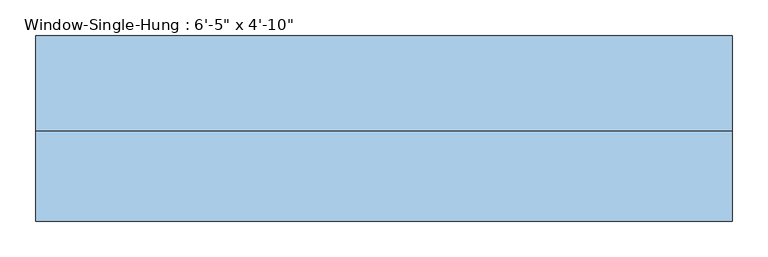
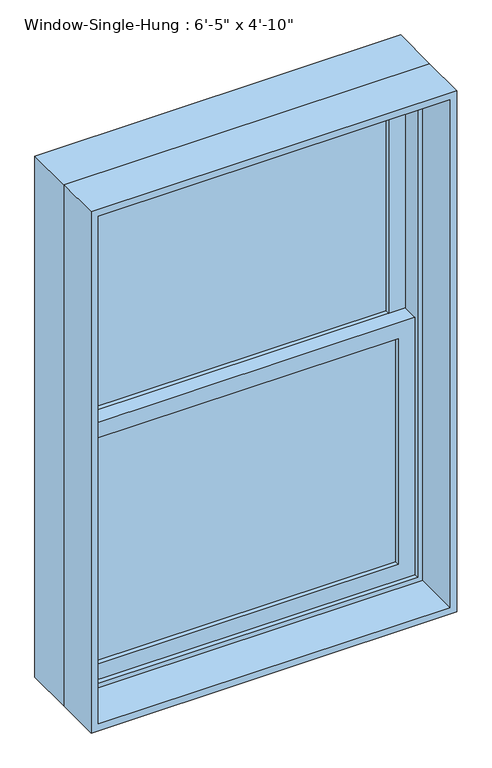
"""IFC4 building model written with IfcOpenShell, lengths in millimetres: window geometry."""

from ifc_helpers import new_model, si_unit, frame, origin, place, context, project, spatial, polyline, outline, extrude, source, transform, mapped, element, save


def window_979dede4(model_context):
    return source(origin(), model_context, "Body", "SweptSolid", [
        extrude(outline(polyline([(412.75, 50.8), (412.75, 44.45), (-412.75, 44.45), (-412.75, 50.8), (412.75, 50.8)])), frame((0.0, 0.0, 990.6), z_axis=(0.0, 0.0, 1.0), x_axis=(1.0, 0.0, 0.0)), (0.0, 0.0, 1.0), 638.175),
        extrude(outline(polyline([(-412.75, 38.1), (412.75, 38.1), (412.75, 31.75), (-412.75, 31.75), (-412.75, 38.1)])), frame((0.0, 0.0, 990.6), z_axis=(0.0, 0.0, 1.0), x_axis=(1.0, 0.0, 0.0)), (0.0, 0.0, 1.0), 638.175),
        extrude(outline(polyline([(412.75, 95.25), (412.75, 88.9), (-412.75, 88.9), (-412.75, 95.25), (412.75, 95.25)])), frame((0.0, 0.0, 1673.225), z_axis=(0.0, 0.0, 1.0), x_axis=(1.0, 0.0, 0.0)), (0.0, 0.0, 1.0), 638.175),
        extrude(outline(polyline([(-412.75, 82.55), (412.75, 82.55), (412.75, 76.2), (-412.75, 76.2), (-412.75, 82.55)])), frame((0.0, 0.0, 1673.225), z_axis=(0.0, 0.0, 1.0), x_axis=(1.0, 0.0, 0.0)), (0.0, 0.0, 1.0), 638.175),
        extrude(outline(polyline([(1673.225, -457.2), (946.15, -457.2), (946.15, 457.2), (1673.225, 457.2), (1673.225, -457.2)]), holes=[polyline([(1628.775, 412.75), (990.6, 412.75), (990.6, -412.75), (1628.775, -412.75), (1628.775, 412.75)])]), frame((0.0, 19.05, 0.0), z_axis=(0.0, 1.0, 0.0), x_axis=(0.0, 0.0, 1.0)), (0.0, 0.0, 1.0), 44.45),
        extrude(outline(polyline([(2355.85, -457.2), (1628.775, -457.2), (1628.775, 457.2), (2355.85, 457.2), (2355.85, -457.2)]), holes=[polyline([(2311.4, 412.75), (1673.225, 412.75), (1673.225, -412.75), (2311.4, -412.75), (2311.4, 412.75)])]), frame((0.0, 63.5, 0.0), z_axis=(0.0, 1.0, 0.0), x_axis=(0.0, 0.0, 1.0)), (0.0, 0.0, 1.0), 44.45),
        extrude(outline(polyline([(2387.6, -488.95), (914.4, -488.95), (914.4, 488.95), (2387.6, 488.95), (2387.6, -488.95)]), holes=[polyline([(2355.85, 457.2), (946.15, 457.2), (946.15, -457.2), (2355.85, -457.2), (2355.85, 457.2)])]), frame((0.0, 6.35, 0.0), z_axis=(0.0, 1.0, 0.0), x_axis=(0.0, 0.0, 1.0)), (0.0, 0.0, 1.0), 133.35),
        extrude(outline(polyline([(2387.6, 488.95), (2387.6, -488.95), (914.4, -488.95), (914.4, 488.95), (2387.6, 488.95)]), holes=[polyline([(2368.55, 469.9), (933.45, 469.9), (933.45, -469.9), (2368.55, -469.9), (2368.55, 469.9)])]), frame((0.0, -120.65, 0.0), z_axis=(0.0, 1.0, 0.0), x_axis=(0.0, 0.0, 1.0)), (0.0, 0.0, 1.0), 127.0),
    ])


if __name__ == "__main__":
    model = new_model("IFC4")
    model_context = context("Model", 3, world=origin())
    ifc_project = project(units=[si_unit("LENGTHUNIT", "METRE", prefix="MILLI")], contexts=[model_context])
    site = spatial("IfcSite", under=ifc_project)
    building = spatial("IfcBuilding", under=site)
    placement = place(None, origin())
    window_shape = window_979dede4(model_context)
    element("IfcWindow", 1, ObjectType="Window-Single-Hung : 6'-5\" x 4'-10\"", at=placement, inside=building, context=model_context, shape_type="MappedRepresentation", body=[
        mapped(window_shape, transform((0.0, 0.0, 0.0), x_axis=(1.0, 0.0, 0.0), y_axis=(0.0, 1.0, 0.0), z_axis=(0.0, 0.0, 1.0))),
    ])
    save(model, "model.ifc")

# Revit data of these elements
# Type "Window-Single-Hung : 6'-5\" x 4'-10\""
#   Type Mark = "19"
#   Fire Rating = "0.5h"
#   Construction Type Id = "DG-DR"
#   Assembly Code = "B2020100"
#   Analytic Construction = "Double glazing - domestic"
#   Wall Thickness [instance default] = 0' - 6"
#   Window Inset [instance default] = 0' - 0"
#   Visual Light Transmittance = 0.81
#   Thermal Resistance (R) = 0.319569 (m²·K)/W
#   Solar Heat Gain Coefficient = 0.76
#   Muntin Width = 2' - 8 1/2"
#   Muntin Height = 2' - 1 1/8"
#   Interior Wall Closure [instance default] = 0' - 1 1/2"
#   Rough Width = 3' - 3"
#   Rough Height = 4' - 10 1/2"
#   Frame Extension [instance default] = 0' - 1 1/4"
#   Exterior Wall Closure [instance default] = 0' - 0 1/2"
#   Extension Jamb [instance default] = 0' - 1 1/2"
#   Heat Transfer Coefficient (U) = 3.12929 W/(m²·K)
#   Height = 4' - 10"
#   Width = 3' - 2 1/2"
#   Top Muntin Visibility = no
#   Indicator Visibility = no
#   Extension Jamb Visibility [instance default] = yes
#   Interior Trim Visibility [instance default] = yes
#   Exterior Trim Visibility [instance default] = yes
#   Bottom Muntin Visibility = no
#   Muntin Pattern = Muntin Pattern_2x2 : Muntin Pattern_2x2
#   Interior Trim Material = Wood - Stained
#   Interior Trim = Trim-Window-Interior-Flat : Picture Frame
#   Exterior Trim Material = Clad - White
#   Exterior Trim = Trim-Window-Exterior-Flat : with Sill
#   Glass Panel Material = Glass
#   Exterior Frame Material = Clad - White
#   Interior Frame Material = Wood - Stained
#   Wall Closure = (empty or 0)
# Element 1 (IfcWindow, "Window-Single-Hung : 6'-5\" x 4'-10\"")
#   Wall Thickness = 0' - 9 1/2"
#   Extension Jamb = 0' - 5"
#   Materials on its faces: "Wood - Stained", "Glass", "Clad - White"
# Materials
#   "Wood - Stained": class "Wood", colour RGB 224 178 126, transparency 0, Cost = 0
#   "Clad - White": class "Wood", colour RGB 242 242 238, transparency 0, Cost = 0
#   "Glass": class "Glass", colour RGB 218 227 224, transparency 0.85, Description = "Soda Lime Glass", Cost = 0
